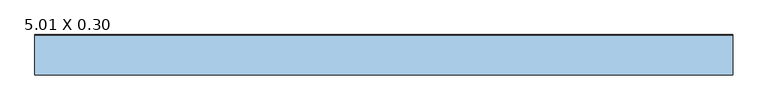
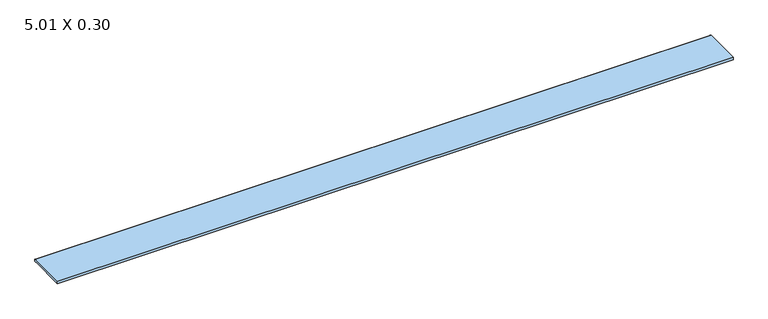
"""IFC4 building model written with IfcOpenShell, lengths in millimetres: window geometry, .CC_ND 300_PEDRA_PEITORIL RETO : 5.01 X 0.30."""

from ifc_helpers import new_model, si_unit, point, frame, frame_2d, origin, place, context, project, spatial, polyline, circle_curve, trimmed, segment, composite_curve, outline, extrude, source, transform, mapped, element, save


def window_5_01_x_0_30_29a636ee(model_context):
    return source(origin(), model_context, "Body", "SweptSolid", [
        extrude(outline(composite_curve([segment(polyline([(144.4083081, 1480.0), (-129.9, 1480.0), (-129.9, 1500.0), (153.2808343, 1500.0)]), True, "CONTINUOUS"), segment(trimmed(circle_curve(frame_2d((153.2808343, 1493.3808343)), 6.6191657), [point((153.2808343, 1500.0))], [point((159.9, 1493.3808343))], False, "CARTESIAN"), True, "CONTINUOUS"), segment(polyline([(159.9, 1493.3808343), (159.9, 1480.0), (149.1619526, 1480.0), (149.1619526, 1488.1993124), (144.4083081, 1488.1993124), (144.4083081, 1480.0)]), True, "CONTINUOUS")], self_intersect=False)), frame((-2505.0, 0.0, 0.0), z_axis=(1.0, 0.0, 0.0), x_axis=(0.0, 1.0, 0.0)), (0.0, 0.0, 1.0), 5010.0),
    ])


if __name__ == "__main__":
    model = new_model("IFC4")
    model_context = context("Model", 3, world=origin())
    ifc_project = project(units=[si_unit("LENGTHUNIT", "METRE", prefix="MILLI")], contexts=[model_context])
    site = spatial("IfcSite", under=ifc_project)
    building = spatial("IfcBuilding", under=site)
    placement = place(None, origin())
    window_5_01_x_0_30_shape = window_5_01_x_0_30_29a636ee(model_context)
    element("IfcWindow", 1, ObjectType=".CC_ND 300_PEDRA_PEITORIL RETO : 5.01 X 0.30", at=placement, inside=building, context=model_context, shape_type="MappedRepresentation", body=[
        mapped(window_5_01_x_0_30_shape, transform((0.0, 0.0, 0.0), x_axis=(1.0, 0.0, 0.0), y_axis=(0.0, 1.0, 0.0), z_axis=(0.0, 0.0, 1.0))),
    ])
    save(model, "model.ifc")

# Revit data of these elements
# Type ".CC_ND 300_PEDRA_PEITORIL RETO : 5.01 X 0.30"
#   Type Mark = "71"
#   Largura da pedra [instance default] = 0.26 m
#   Extensão interior peitoril [instance default] = 0.03 m
#   Extensão exterior peitoril [instance default] = 0.03 m
#   Espessura = 0.02 m
#   Comprimento = 5.01 m
#   Altura-padrão do peitoril = 1.48 m
#   Peitoril = .GRANITO_BRANCO_ITAUNAS
#   Rough Width = 0
#   Rough Height = 0
#   Height = 0
#   Wall Closure = (empty or 0)
#   Width = 0
# Element 1 (IfcWindow, ".CC_ND 300_PEDRA_PEITORIL RETO : 5.01 X 0.30")
#   Largura da pedra = 0.2898 m
#   Extensão interior peitoril = 0.00 m
#   Materials on its faces: ".GRANITO_BRANCO_ITAUNAS"
# Materials
#   ".GRANITO_BRANCO_ITAUNAS": class ".CC_PEDRA REVEST.", colour RGB 202 195 174, transparency 0, Description = "Revestimento em granito", Cost = 0
